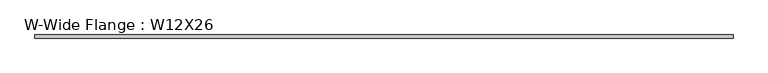
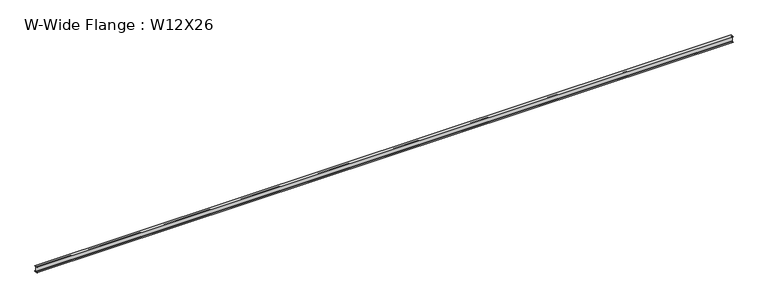
"""IFC4 building model written with IfcOpenShell, lengths in millimetres: beam geometry, W-Wide Flange : W12X26."""

from ifc_helpers import new_model, si_unit, point, frame, frame_2d, origin, place, context, project, spatial, polyline, circle_curve, trimmed, segment, composite_curve, outline, extrude, source, transform, mapped, element, save


def w_wide_flange_w12x26_f67572b3(model_context):
    return source(origin(), model_context, "Body", "SweptSolid", [
        extrude(outline(composite_curve([segment(polyline([(82.4011719, -145.5539063), (82.4011719, -155.178125), (-82.4011719, -155.178125), (-82.4011719, -145.5539063), (-20.2902344, -145.5539063)]), True, "CONTINUOUS"), segment(trimmed(circle_curve(frame_2d((-20.2902344, -128.190625)), 17.3632812), [point((-20.2902344, -145.5539063))], [point((-2.9269531, -128.190625))], True, "CARTESIAN"), True, "CONTINUOUS"), segment(polyline([(-2.9269531, -128.190625), (-2.9269531, 128.190625)]), True, "CONTINUOUS"), segment(trimmed(circle_curve(frame_2d((-20.2902344, 128.190625)), 17.3632812), [point((-2.9269531, 128.190625))], [point((-20.2902344, 145.5539062))], True, "CARTESIAN"), True, "CONTINUOUS"), segment(polyline([(-20.2902344, 145.5539062), (-82.4011719, 145.5539062), (-82.4011719, 155.178125), (82.4011719, 155.178125), (82.4011719, 145.5539062), (20.2902344, 145.5539062)]), True, "CONTINUOUS"), segment(trimmed(circle_curve(frame_2d((20.2902344, 128.190625)), 17.3632812), [point((20.2902344, 145.5539062))], [point((2.9269531, 128.190625))], True, "CARTESIAN"), True, "CONTINUOUS"), segment(polyline([(2.9269531, 128.190625), (2.9269531, -128.190625)]), True, "CONTINUOUS"), segment(trimmed(circle_curve(frame_2d((20.2902344, -128.190625)), 17.3632812), [point((2.9269531, -128.190625))], [point((20.2902344, -145.5539063))], True, "CARTESIAN"), True, "CONTINUOUS"), segment(polyline([(20.2902344, -145.5539063), (82.4011719, -145.5539063)]), True, "CONTINUOUS")], self_intersect=False)), frame((-18489.1180586, 0.0, 0.0), z_axis=(1.0, 0.0, 0.0), x_axis=(0.0, 1.0, 0.0)), (0.0, 0.0, 1.0), 36978.2361173),
    ])


if __name__ == "__main__":
    model = new_model("IFC4")
    model_context = context("Model", 3, world=origin())
    ifc_project = project(units=[si_unit("LENGTHUNIT", "METRE", prefix="MILLI")], contexts=[model_context])
    site = spatial("IfcSite", under=ifc_project)
    building = spatial("IfcBuilding", under=site)
    placement = place(None, origin())
    w_wide_flange_w12x26_shape = w_wide_flange_w12x26_f67572b3(model_context)
    element("IfcBeam", 1, ObjectType="W-Wide Flange : W12X26", at=placement, inside=building, context=model_context, shape_type="MappedRepresentation", body=[
        mapped(w_wide_flange_w12x26_shape, transform((0.0, 0.0, 0.0), x_axis=(1.0, 0.0, 0.0), y_axis=(0.0, 1.0, 0.0), z_axis=(0.0, 0.0, 1.0))),
    ])
    save(model, "model.ifc")

# Revit data of these elements
# Type "W-Wide Flange : W12X26"
#   Assembly Code = "B10"
#   W = 26
#   Length [instance default] = 5' - 0"
#   bf = 0' - 6 125/256"
#   d = 1' - 0 7/32"
#   k = 0' - 1 1/16"
#   k2 = 0' - 0 175/256"
#   tf = 0' - 0 97/256"
#   tw = 0' - 0 59/256"
#   A = 0.053125 SF
#   Structural Material [instance default] = none
